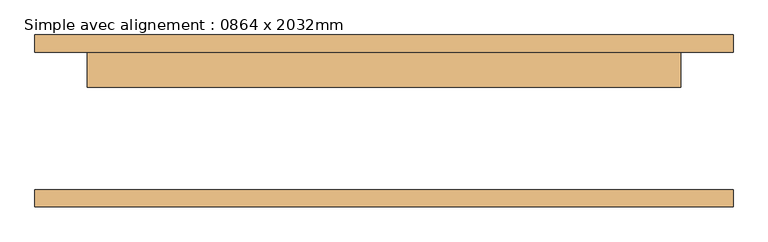
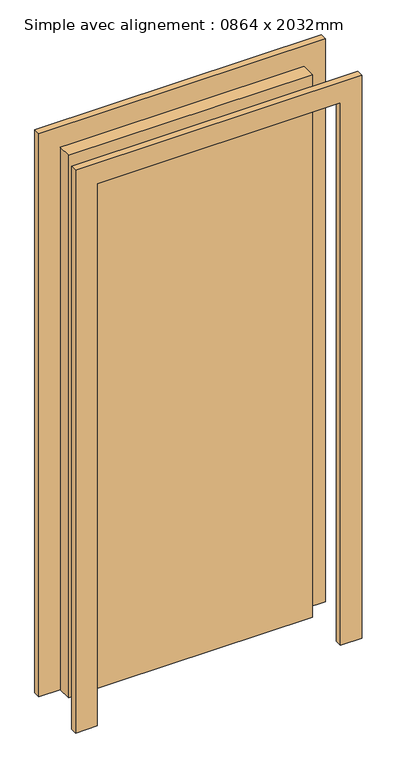
"""IFC4 building model written with IfcOpenShell, lengths in millimetres: door geometry, Simple avec alignement : 0864 x 2032mm."""

from ifc_helpers import new_model, si_unit, frame, origin, origin_with_axes, place, context, project, spatial, polyline, outline, extrude, source, transform, mapped, element, save


def simple_avec_alignement_0864_x_2032mm_aeff3166(model_context):
    return source(origin(), model_context, "Body", "SweptSolid", [
        extrude(outline(polyline([(2108.0, -508.0), (0.0, -508.0), (0.0, -432.0), (2032.0, -432.0), (2032.0, 432.0), (0.0, 432.0), (0.0, 508.0), (2108.0, 508.0), (2108.0, -508.0)])), frame((0.0, 100.0, 0.0), z_axis=(0.0, 1.0, 0.0), x_axis=(0.0, 0.0, 1.0)), (0.0, 0.0, 1.0), 25.0),
        extrude(outline(polyline([(2108.0, 508.0), (2108.0, -508.0), (0.0, -508.0), (0.0, -432.0), (2032.0, -432.0), (2032.0, 432.0), (0.0, 432.0), (0.0, 508.0), (2108.0, 508.0)])), frame((0.0, -125.0, 0.0), z_axis=(0.0, 1.0, 0.0), x_axis=(0.0, 0.0, 1.0)), (0.0, 0.0, 1.0), 25.0),
        extrude(outline(polyline([(432.0, 49.0), (-432.0, 49.0), (-432.0, 100.0), (432.0, 100.0), (432.0, 49.0)])), origin_with_axes(), (0.0, 0.0, 1.0), 2032.0),
    ])


if __name__ == "__main__":
    model = new_model("IFC4")
    model_context = context("Model", 3, world=origin())
    ifc_project = project(units=[si_unit("LENGTHUNIT", "METRE", prefix="MILLI")], contexts=[model_context])
    site = spatial("IfcSite", under=ifc_project)
    building = spatial("IfcBuilding", under=site)
    placement = place(None, origin())
    simple_avec_alignement_0864_x_2032mm_shape = simple_avec_alignement_0864_x_2032mm_aeff3166(model_context)
    element("IfcDoor", 1, ObjectType="Simple avec alignement : 0864 x 2032mm", at=placement, inside=building, context=model_context, shape_type="MappedRepresentation", body=[
        mapped(simple_avec_alignement_0864_x_2032mm_shape, transform((0.0, 0.0, 0.0), x_axis=(1.0, 0.0, 0.0), y_axis=(0.0, 1.0, 0.0), z_axis=(0.0, 0.0, 1.0))),
    ])
    save(model, "model.ifc")

# Revit data of these elements
# Type "Simple avec alignement : 0864 x 2032mm"
#   Type Mark = "22"
#   Construction Type Id = "MDOOR"
#   Analytic Construction = "Métal"
#   Thickness = 0.051 m
#   Heat Transfer Coefficient (U) = 3.7021 W/(m²·K)
#   Height = 2.032 m
#   Ajuster la projection Ext = 0.025 m
#   Ajuster la projection Int = 0.025 m
#   Ajuster la largeur = 0.076 m
#   Width = 0.864 m
#   Function = 0
#   Define Thermal Properties by = 1
#   Matériau de porte = Porte - Panneau
#   Matériau des huisseries = Porte - Cadre
#   Visual Light Transmittance = 0
#   Solar Heat Gain Coefficient = 0
#   Function = (empty or 0)
#   Wall Closure = (empty or 0)
# Element 1 (IfcDoor, "Simple avec alignement : 0864 x 2032mm")
#   Materials on its faces: "Porte - Cadre", "Porte - Panneau"
# Materials
#   "Porte - Panneau": class "Bois", colour RGB 210 159 95, transparency 0, Cost = 0
#   "Porte - Cadre": class "Peinture", colour RGB 118 70 51, transparency 0, Cost = 0
